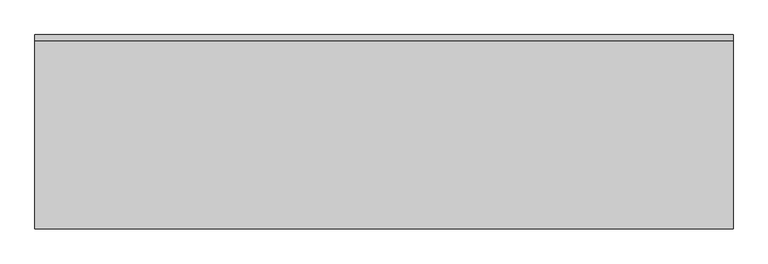
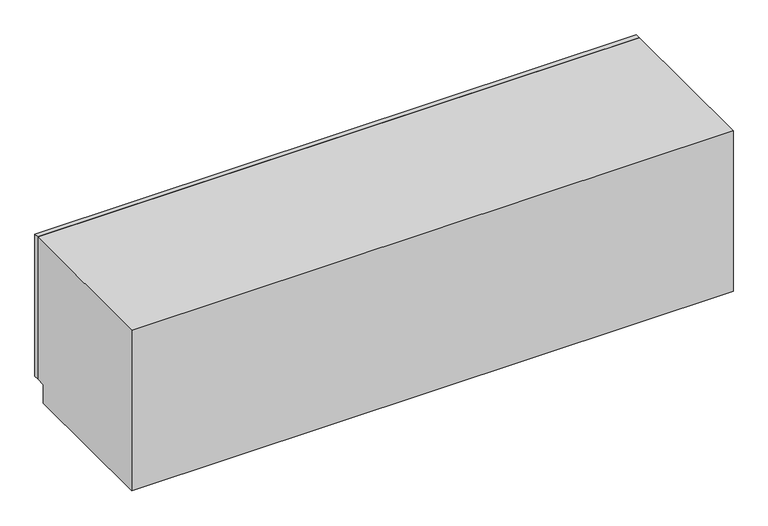
"""IFC4 building model written with IfcOpenShell, lengths in millimetres: furniture geometry, OD_CW_Base Cabinet : OD_CW_Base Cabinet."""

from ifc_helpers import new_model, si_unit, frame, origin, place, context, project, spatial, polyline, outline, extrude, source, transform, mapped, element, save


def furniture_c5d2c231(model_context):
    return source(origin(), model_context, "Body", "SweptSolid", [
        extrude(outline(polyline([(18.7377049, 228.6), (18.7377049, 254.0), (3123.5891463, 254.0), (3123.5891463, 228.6), (18.7377049, 228.6)])), frame((0.0, 0.0, 101.6), z_axis=(0.0, 0.0, 1.0), x_axis=(1.0, 0.0, 0.0)), (0.0, 0.0, 1.0), 774.7),
        extrude(outline(polyline([(228.6, 876.3), (228.6, 101.6), (177.8, 101.6), (177.8, 0.0), (-609.6, 0.0), (-609.6, 876.3), (228.6, 876.3)])), frame((18.7377049, 0.0, 0.0), z_axis=(1.0, 0.0, 0.0), x_axis=(0.0, 1.0, 0.0)), (0.0, 0.0, 1.0), 3104.8514414),
    ])


if __name__ == "__main__":
    model = new_model("IFC4")
    model_context = context("Model", 3, world=origin())
    ifc_project = project(units=[si_unit("LENGTHUNIT", "METRE", prefix="MILLI")], contexts=[model_context])
    site = spatial("IfcSite", under=ifc_project)
    building = spatial("IfcBuilding", under=site)
    placement = place(None, origin())
    furniture_shape = furniture_c5d2c231(model_context)
    element("IfcFurniture", 1, ObjectType="OD_CW_Base Cabinet : OD_CW_Base Cabinet", at=placement, inside=building, context=model_context, shape_type="MappedRepresentation", body=[
        mapped(furniture_shape, transform((0.0, 0.0, 0.0), x_axis=(1.0, 0.0, 0.0), y_axis=(0.0, 1.0, 0.0), z_axis=(0.0, 0.0, 1.0))),
    ])
    save(model, "model.ifc")

# Revit data of these elements
# Type "OD_CW_Base Cabinet : OD_CW_Base Cabinet"
#   OD_CW_Width [instance default] = 2' - 10"
#   OD_CW_Length [instance default] = 8' - 0"
#   OD_CW_Height [instance default] = 2' - 3"
#   Depth = 2' - 0"
#   Height = 3' - 0"
#   Width = 4' - 0"
#   OD_CW_Material_Front Panel [instance default] = none
#   OD_CW_Material_Body [instance default] = none
# Element 1 (IfcFurniture, "OD_CW_Base Cabinet : OD_CW_Base Cabinet")
#   OD_CW_Length = 10' - 2.23825"
#   OD_CW_Height = 2' - 10 1/2"
#   OD_CW_Material_Front Panel = WOOD-OAKFIRE
#   OD_CW_Material_Body = WOOD-OAKFIRE
#   Materials on its faces: "WOOD-OAKFIRE"
# Materials
#   "WOOD-OAKFIRE": class "Wood", colour RGB 198 202 183, transparency 0, Description = "Generic wood", Cost = 0
